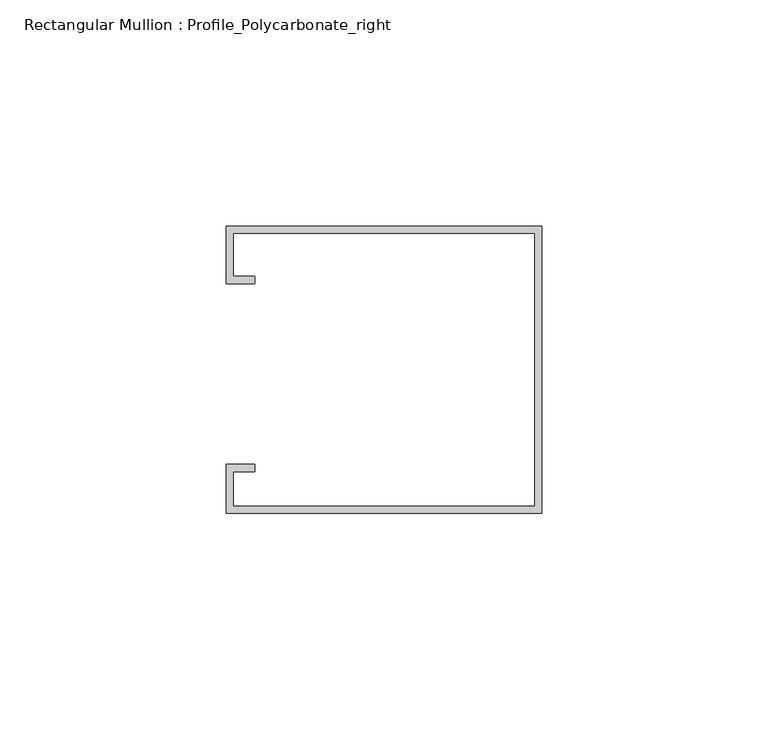
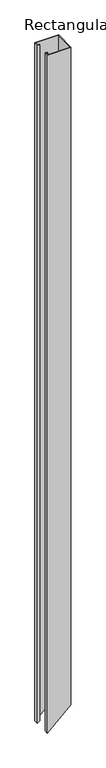
"""IFC4 building model written with IfcOpenShell, lengths in millimetres: member geometry, Rectangular Mullion : Profile_Polycarbonate_right."""

from ifc_helpers import new_model, si_unit, origin, place, context, project, spatial, faceted_brep, source, transform, mapped, element, save


def rectangular_mullion_profile_polycarbonate_right_72364b00(model_context):
    return source(origin(), model_context, "Body", "Brep", [
        faceted_brep([(0.0, 32.7, 0.0), (-69.85, 32.7, 0.0), (-69.85, 20.0, 0.0), (-63.5, 20.0, 0.0), (-63.5, 21.5875, 0.0), (-68.2625, 21.5875, 0.0), (-68.2625, 31.1125, 0.0), (-1.5875, 31.1125, 0.0), (-1.5875, -29.2125, 0.0), (-68.2625, -29.2125, 0.0), (-68.2625, -21.5875, 0.0), (-63.5, -21.5875, 0.0), (-63.5, -20.0, 0.0), (-69.85, -20.0, 0.0), (-69.85, -30.8, 0.0), (0.0, -30.8, 0.0), (0.0, 32.7, -2051.5791667), (-69.85, 32.7, -2115.8504484), (-69.85, 20.0, -2115.8504484), (-63.5, 20.0, -2110.0076046), (-63.5, 21.5875, -2110.0076046), (-68.2625, 21.5875, -2114.3897375), (-68.2625, 31.1125, -2114.3897375), (-1.5875, 31.1125, -2053.0398776), (-1.5875, -29.2125, -2053.0398776), (-68.2625, -29.2125, -2114.3897375), (-68.2625, -21.5875, -2114.3897375), (-63.5, -21.5875, -2110.0076046), (-63.5, -20.0, -2110.0076046), (-69.85, -20.0, -2115.8504484), (-69.85, -30.8, -2115.8504484), (0.0, -30.8, -2051.5791667)], [[[0, 1, 2, 3, 4, 5, 6, 7, 8, 9, 10, 11, 12, 13, 14, 15]], [[1, 0, 16, 17]], [[2, 1, 17, 18]], [[3, 2, 18, 19]], [[4, 3, 19, 20]], [[5, 4, 20, 21]], [[6, 5, 21, 22]], [[7, 6, 22, 23]], [[8, 7, 23, 24]], [[9, 8, 24, 25]], [[10, 9, 25, 26]], [[11, 10, 26, 27]], [[12, 11, 27, 28]], [[13, 12, 28, 29]], [[14, 13, 29, 30]], [[15, 14, 30, 31]], [[0, 15, 31, 16]], [[16, 31, 30, 29, 28, 27, 26, 25, 24, 23, 22, 21, 20, 19, 18, 17]]]),
    ])


if __name__ == "__main__":
    model = new_model("IFC4")
    model_context = context("Model", 3, world=origin())
    ifc_project = project(units=[si_unit("LENGTHUNIT", "METRE", prefix="MILLI")], contexts=[model_context])
    site = spatial("IfcSite", under=ifc_project)
    building = spatial("IfcBuilding", under=site)
    placement = place(None, origin())
    rectangular_mullion_profile_polycarbonate_right_shape = rectangular_mullion_profile_polycarbonate_right_72364b00(model_context)
    element("IfcMember", 1, ObjectType="Rectangular Mullion : Profile_Polycarbonate_right", at=placement, inside=building, context=model_context, shape_type="MappedRepresentation", body=[
        mapped(rectangular_mullion_profile_polycarbonate_right_shape, transform((0.0, 0.0, 0.0), x_axis=(1.0, 0.0, 0.0), y_axis=(0.0, 1.0, 0.0), z_axis=(0.0, 0.0, 1.0))),
    ])
    save(model, "model.ifc")

# Revit data of these elements
# Type "Rectangular Mullion : Profile_Polycarbonate_right"
#   built-in parameter 1007322 = 0.208333 (stored number, unit not read)
#   built-in parameter 1007321 = 0 (stored number, unit not read)
#   built-in parameter 1007320 = 0.00520833 (stored number, unit not read)
# Element 1 (IfcMember, "Rectangular Mullion : Profile_Polycarbonate_right")
#   Materials on its faces: "ALUMINUM PROFILE AT POLYCARBONATE PANEL"
# Materials
#   "ALUMINUM PROFILE AT POLYCARBONATE PANEL": class "Metal", colour RGB 244 244 244, transparency 0, Description = "Aluminum 6061", Cost = 0
